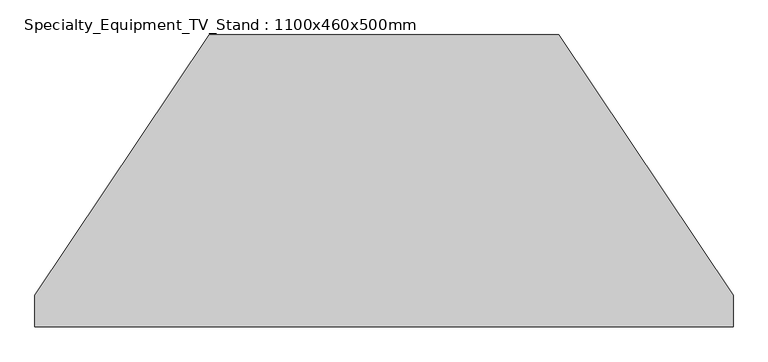
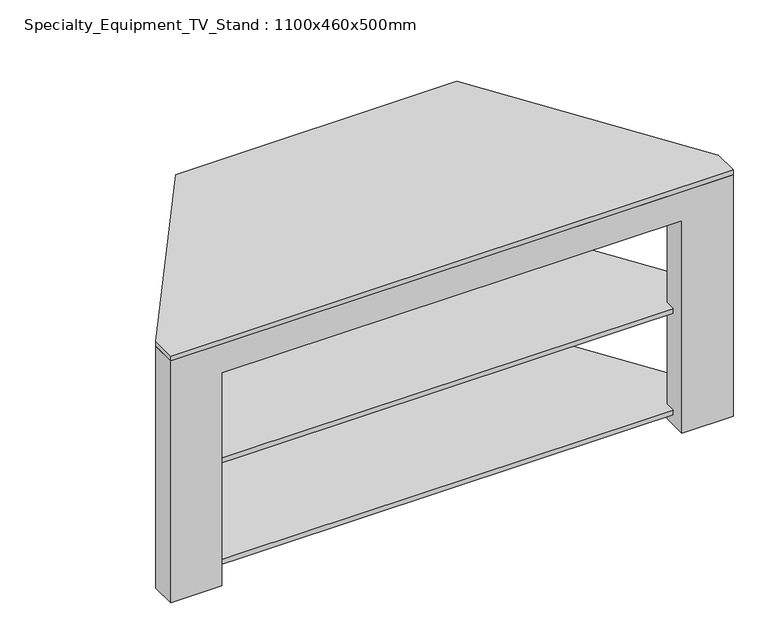
"""IFC4 building model written with IfcOpenShell, lengths in millimetres: proxy geometry, Specialty_Equipment_TV_Stand : 1100x460x500mm."""

from ifc_helpers import new_model, si_unit, point, frame, frame_2d, origin, place, context, project, spatial, polyline, circle_curve, trimmed, segment, composite_curve, outline, extrude, faceted_brep, source, transform, mapped, element, save


def specialty_equipment_tv_stand_1100x460x500mm_40ec15d9(model_context):
    return source(origin(), model_context, "Body", "SolidModel", [
        extrude(outline(polyline([(420.3099533, -30.0), (625.1880021, -335.4545455), (625.1880021, -430.0), (-374.8119979, -430.0), (-374.8119979, -335.4545455), (-169.9339492, -30.0), (420.3099533, -30.0)])), frame((0.0, 0.0, 20.0), z_axis=(0.0, 0.0, 1.0), x_axis=(1.0, 0.0, 0.0)), (0.0, 0.0, 1.0), 10.0),
        extrude(outline(polyline([(420.3099533, -30.0), (625.1880021, -335.4545455), (625.1880021, -430.0), (-374.8119979, -430.0), (-374.8119979, -335.4545455), (-169.9339492, -30.0), (420.3099533, -30.0)])), frame((0.0, 0.0, 230.0), z_axis=(0.0, 0.0, 1.0), x_axis=(1.0, 0.0, 0.0)), (0.0, 0.0, 1.0), 10.0),
        extrude(outline(polyline([(400.1880021, 0.0), (675.1880021, -410.0), (675.1880021, -460.0), (-424.8119979, -460.0), (-424.8119979, -410.0), (-149.8119979, 0.0), (400.1880021, 0.0)])), frame((0.0, 0.0, 500.0), z_axis=(0.0, 0.0, 1.0), x_axis=(1.0, 0.0, 0.0)), (0.0, 0.0, 1.0), 10.0),
        extrude(outline(polyline([(-50.0, 500.0), (0.0, 500.0), (0.0, 0.0), (-50.0, 0.0), (-50.0, 20.0), (-30.0, 20.0), (-30.0, 30.0), (-50.0, 30.0), (-50.0, 230.0), (-30.0, 230.0), (-30.0, 240.0), (-50.0, 240.0), (-50.0, 500.0)])), frame((-149.8119979, 0.0, 0.0), z_axis=(1.0, 0.0, 0.0), x_axis=(0.0, 1.0, 0.0)), (0.0, 0.0, 1.0), 100.0),
        extrude(outline(polyline([(-50.0, 500.0), (0.0, 500.0), (0.0, 0.0), (-50.0, 0.0), (-50.0, 20.0), (-30.0, 20.0), (-30.0, 30.0), (-50.0, 30.0), (-50.0, 230.0), (-30.0, 230.0), (-30.0, 240.0), (-50.0, 240.0), (-50.0, 500.0)])), frame((300.1880021, 0.0, 0.0), z_axis=(1.0, 0.0, 0.0), x_axis=(0.0, 1.0, 0.0)), (0.0, 0.0, 1.0), 100.0),
        faceted_brep([(-424.8119979, -460.0, 0.0), (-324.8119979, -460.0, 0.0), (-324.8119979, -460.0, 440.0), (575.1880021, -460.0, 440.0), (575.1880021, -460.0, 0.0), (675.1880021, -460.0, 0.0), (675.1880021, -460.0, 500.0), (-424.8119979, -460.0, 500.0), (-424.8119979, -410.0, 0.0), (-424.8119979, -410.0, 500.0), (675.1880021, -410.0, 500.0), (675.1880021, -410.0, 0.0), (575.1880021, -410.0, 0.0), (575.1880021, -410.0, 20.0), (625.1880021, -410.0, 20.0), (625.1880021, -410.0, 30.0), (575.1880021, -410.0, 30.0), (575.1880021, -410.0, 230.0), (625.1880021, -410.0, 230.0), (625.1880021, -410.0, 240.0), (575.1880021, -410.0, 240.0), (575.1880021, -410.0, 440.0), (-324.8119979, -410.0, 440.0), (-324.8119979, -410.0, 240.0), (-374.8119979, -410.0, 240.0), (-374.8119979, -410.0, 230.0), (-324.8119979, -410.0, 230.0), (-324.8119979, -410.0, 30.0), (-374.8119979, -410.0, 30.0), (-374.8119979, -410.0, 20.0), (-324.8119979, -410.0, 20.0), (-324.8119979, -410.0, 0.0), (-324.8119979, -430.0, 20.0), (-324.8119979, -430.0, 30.0), (-324.8119979, -430.0, 230.0), (-324.8119979, -430.0, 240.0), (575.1880021, -430.0, 240.0), (575.1880021, -430.0, 230.0), (575.1880021, -430.0, 30.0), (575.1880021, -430.0, 20.0), (625.1880021, -430.0, 240.0), (-374.8119979, -430.0, 240.0), (-374.8119979, -430.0, 230.0), (625.1880021, -430.0, 230.0), (625.1880021, -430.0, 30.0), (-374.8119979, -430.0, 30.0), (-374.8119979, -430.0, 20.0), (625.1880021, -430.0, 20.0)], [[[0, 1, 2, 3, 4, 5, 6, 7]], [[8, 9, 10, 11, 12, 13, 14, 15, 16, 17, 18, 19, 20, 21, 22, 23, 24, 25, 26, 27, 28, 29, 30, 31]], [[1, 0, 8, 31]], [[2, 1, 31, 30, 32, 33, 27, 26, 34, 35, 23, 22]], [[3, 2, 22, 21]], [[4, 3, 21, 20, 36, 37, 17, 16, 38, 39, 13, 12]], [[5, 4, 12, 11]], [[6, 5, 11, 10]], [[7, 6, 10, 9]], [[0, 7, 9, 8]], [[19, 40, 36, 20]], [[35, 41, 24, 23]], [[25, 42, 34, 26]], [[37, 43, 18, 17]], [[41, 42, 25, 24]], [[42, 41, 35, 34]], [[40, 43, 37, 36]], [[43, 40, 19, 18]], [[15, 44, 38, 16]], [[33, 45, 28, 27]], [[29, 46, 32, 30]], [[39, 47, 14, 13]], [[45, 46, 29, 28]], [[46, 45, 33, 32]], [[44, 47, 39, 38]], [[47, 44, 15, 14]]]),
        extrude(outline(polyline([(0.0, 300.1880021), (500.0, 300.1880021), (500.0, -49.8119979), (0.0, -49.8119979), (0.0, 300.1880021)]), holes=[composite_curve([segment(polyline([(245.0, 145.1700818), (245.0, 105.2059224)]), True, "CONTINUOUS"), segment(trimmed(circle_curve(frame_2d((257.5, 105.2059224)), 12.5), [point((245.0, 105.2059224))], [point((270.0, 105.2059224))], True, "CARTESIAN"), True, "CONTINUOUS"), segment(polyline([(270.0, 105.2059224), (270.0, 145.1700818)]), True, "CONTINUOUS"), segment(trimmed(circle_curve(frame_2d((257.5, 145.1700818)), 12.5), [point((270.0, 145.1700818))], [point((245.0, 145.1700818))], True, "CARTESIAN"), True, "CONTINUOUS")], self_intersect=False), composite_curve([segment(polyline([(35.0, 145.1880021), (35.0, 105.2059224)]), True, "CONTINUOUS"), segment(trimmed(circle_curve(frame_2d((47.5, 105.2059224)), 12.5), [point((35.0, 105.2059224))], [point((60.0, 105.2059224))], True, "CARTESIAN"), True, "CONTINUOUS"), segment(polyline([(60.0, 105.2059224), (60.0, 145.1880021)]), True, "CONTINUOUS"), segment(trimmed(circle_curve(frame_2d((47.5, 145.1880021)), 12.5), [point((60.0, 145.1880021))], [point((35.0, 145.1880021))], True, "CARTESIAN"), True, "CONTINUOUS")], self_intersect=False)]), frame((0.0, -30.0, 0.0), z_axis=(0.0, 1.0, 0.0), x_axis=(0.0, 0.0, 1.0)), (0.0, 0.0, 1.0), 10.0),
    ])


if __name__ == "__main__":
    model = new_model("IFC4")
    model_context = context("Model", 3, world=origin())
    ifc_project = project(units=[si_unit("LENGTHUNIT", "METRE", prefix="MILLI")], contexts=[model_context])
    site = spatial("IfcSite", under=ifc_project)
    building = spatial("IfcBuilding", under=site)
    placement = place(None, origin())
    specialty_equipment_tv_stand_1100x460x500mm_shape = specialty_equipment_tv_stand_1100x460x500mm_40ec15d9(model_context)
    element("IfcBuildingElementProxy", 1, Name="Specialty_Equipment_TV_Stand : 1100x460x500mm", ObjectType="Specialty_Equipment_TV_Stand : 1100x460x500mm", at=placement, inside=building, context=model_context, shape_type="MappedRepresentation", body=[
        mapped(specialty_equipment_tv_stand_1100x460x500mm_shape, transform((0.0, 0.0, 0.0), x_axis=(1.0, 0.0, 0.0), y_axis=(0.0, 1.0, 0.0), z_axis=(0.0, 0.0, 1.0))),
    ])
    save(model, "model.ifc")

# Revit data of these elements
# Type "Specialty_Equipment_TV_Stand : 1100x460x500mm"
#   Depth = 460 mm
#   Width = 1100 mm
#   Height = 500 mm
#   Finish = Melamine - Gray
#   Default Elevation = 0
# Element 1 (IfcBuildingElementProxy, "Specialty_Equipment_TV_Stand : 1100x460x500mm")
#   Materials on its faces: "Melamine - Gray", "Glass - Shelves"
# Materials
#   "Melamine - Gray": class "Wood", colour RGB 49 49 49, transparency 0
#   "Glass - Shelves": class "Glass", colour RGB 167 167 167, transparency 0.9
